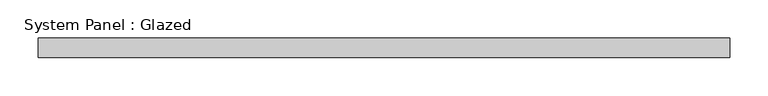
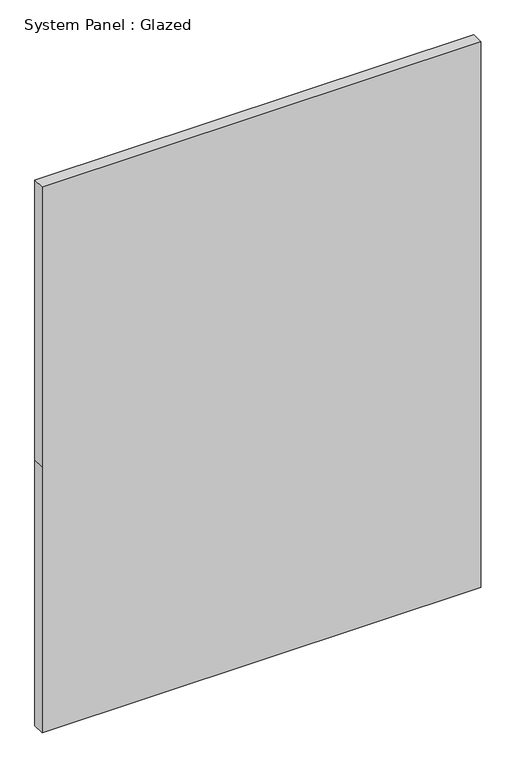
"""IFC4 building model written with IfcOpenShell, lengths in millimetres: plate geometry, System Panel : Glazed."""

import ifcopenshell
import ifcopenshell.guid

model = None  # the IFC model being written
_history = None  # IfcOwnerHistory: only IFC2X3 demands one
_inside = {}  # id of a spatial element -> (the spatial element, [elements in it])
_under = {}  # id of a project, library or spatial element -> (it, [spatial elements below it])
_declared = {}  # id of a project -> (the project, [libraries it declares])
_typed = {}  # id of a type object -> (the type object, [elements of that type])
_made_of = {}  # id of a material, layer set ... -> (it, [elements and type objects made of it])


def new_model(schema):
    """Start an empty IFC model of exactly this schema.

    Asked for "IFC4X3", IfcOpenShell would pick the latest addendum, in which some entities
    have other attributes; the version numbers below select the first issue.
    IFC2X3 requires an IfcOwnerHistory on every rooted entity: one is made here for all.
    """
    global model, _history
    if schema == "IFC4X3":
        model = ifcopenshell.file(schema_version=(4, 3, 0, 0))
    else:
        model = ifcopenshell.file(schema=schema)
    _inside.clear()
    _under.clear()
    _declared.clear()
    _typed.clear()
    _made_of.clear()
    _history = None
    if model.schema == "IFC2X3":
        org = make("IfcOrganization", Name="unknown")
        user = make(
            "IfcPersonAndOrganization",
            ThePerson=make("IfcPerson", FamilyName="unknown"),
            TheOrganization=org,
        )
        app = make(
            "IfcApplication",
            ApplicationDeveloper=org,
            Version="unknown",
            ApplicationFullName="unknown",
            ApplicationIdentifier="unknown",
        )
        _history = make(
            "IfcOwnerHistory",
            OwningUser=user,
            OwningApplication=app,
            ChangeAction="ADDED",
            CreationDate=0,
        )
    return model


def make(cls, **values):
    """One entity of the class cls with the attributes given. An attribute that is None is left unset."""
    return model.create_entity(
        cls, **{name: value for name, value in values.items() if value is not None}
    )


def rooted(cls, **values):
    """An entity with a GlobalId (a new one), such as an element, a storey or a relation."""
    return make(cls, GlobalId=ifcopenshell.guid.new(), OwnerHistory=_history, **values)


def si_unit(unit_type, name, prefix=None):
    """IfcSIUnit, for example si_unit("LENGTHUNIT", "METRE", prefix="MILLI")."""
    return make("IfcSIUnit", UnitType=unit_type, Prefix=prefix, Name=name)


def assignment(units):
    """IfcUnitAssignment: the units of a project."""
    return None if units is None else make("IfcUnitAssignment", Units=units)


def point(xyz):
    """IfcCartesianPoint."""
    return None if xyz is None else make("IfcCartesianPoint", Coordinates=xyz)


def direction(xyz):
    """IfcDirection."""
    return None if xyz is None else make("IfcDirection", DirectionRatios=xyz)


def frame(location, z_axis=None, x_axis=None):
    """IfcAxis2Placement3D, a coordinate frame: its origin and axes. An axis left out is left unset."""
    return make(
        "IfcAxis2Placement3D",
        Location=point(location),
        Axis=direction(z_axis),
        RefDirection=direction(x_axis),
    )


def origin():
    """The frame at (0, 0, 0) with its axes left unset."""
    return frame((0.0, 0.0, 0.0))


def place(relative_to, where):
    """IfcLocalPlacement: puts the frame where relative to a parent placement (None: the world)."""
    return make(
        "IfcLocalPlacement", PlacementRelTo=relative_to, RelativePlacement=where
    )


def context(
    kind, dimensions, precision=None, world=None, true_north=None, identifier=None
):
    """IfcGeometricRepresentationContext, for example the 3D "Model" context."""
    return make(
        "IfcGeometricRepresentationContext",
        ContextIdentifier=identifier,
        ContextType=kind,
        CoordinateSpaceDimension=dimensions,
        Precision=precision,
        WorldCoordinateSystem=world,
        TrueNorth=true_north,
    )


def project(units=None, contexts=None):
    """IfcProject with its units and contexts."""
    return rooted(
        "IfcProject",
        Name="project",
        RepresentationContexts=contexts,
        UnitsInContext=assignment(units),
    )


def spatial(cls, under=None, at=None, **own):
    """A site, building, storey or space (cls), placed at a placement, below another one or the project."""
    s = rooted(cls, ObjectPlacement=at, **own)
    if under is not None:
        _under.setdefault(under.id(), (under, []))[1].append(s)
    return s


def polyline(points):
    """IfcPolyline through the points."""
    return make("IfcPolyline", Points=[point(p) for p in points])


def outline(outer, holes=None, kind="AREA"):
    """IfcArbitraryClosedProfileDef: a profile drawn as a closed curve; with holes, ...WithVoids."""
    if holes is None:
        return make("IfcArbitraryClosedProfileDef", ProfileType=kind, OuterCurve=outer)
    return make(
        "IfcArbitraryProfileDefWithVoids",
        ProfileType=kind,
        OuterCurve=outer,
        InnerCurves=holes,
    )


def extrude(swept, where, along, depth):
    """IfcExtrudedAreaSolid: the profile swept, set in the frame where, extruded along a direction by depth."""
    return make(
        "IfcExtrudedAreaSolid",
        SweptArea=swept,
        Position=where,
        ExtrudedDirection=direction(along),
        Depth=depth,
    )


def shape(context_of_items, identifier, shape_type, items):
    """IfcShapeRepresentation: the items that make up one representation, for example the "Body"."""
    return make(
        "IfcShapeRepresentation",
        ContextOfItems=context_of_items,
        RepresentationIdentifier=identifier,
        RepresentationType=shape_type,
        Items=items,
    )


def source(mapping_origin, context_of_items, identifier, shape_type, items):
    """IfcRepresentationMap: a shape defined once, which mapped items show again and again."""
    return make(
        "IfcRepresentationMap",
        MappingOrigin=mapping_origin,
        MappedRepresentation=shape(context_of_items, identifier, shape_type, items),
    )


def transform(
    local_origin,
    x_axis=None,
    y_axis=None,
    z_axis=None,
    scale=None,
    scale2=None,
    scale3=None,
    uniform=True,
):
    """IfcCartesianTransformationOperator3D, or its non-uniform kind. x_axis, y_axis, z_axis: its Axis1, 2, 3."""
    if uniform:
        return make(
            "IfcCartesianTransformationOperator3D",
            Axis1=direction(x_axis),
            Axis2=direction(y_axis),
            LocalOrigin=point(local_origin),
            Scale=scale,
            Axis3=direction(z_axis),
        )
    return make(
        "IfcCartesianTransformationOperator3DnonUniform",
        Axis1=direction(x_axis),
        Axis2=direction(y_axis),
        LocalOrigin=point(local_origin),
        Scale=scale,
        Axis3=direction(z_axis),
        Scale2=scale2,
        Scale3=scale3,
    )


def mapped(mapping_source, mapping_target):
    """IfcMappedItem: shows the shape of a source again, moved by a transform."""
    return make(
        "IfcMappedItem", MappingSource=mapping_source, MappingTarget=mapping_target
    )


def made_of(thing, what):
    """Note that an element or type object is made of a material, layer set ...; save() writes the relation."""
    if what is not None:
        _made_of.setdefault(what.id(), (what, []))[1].append(thing)
    return thing


def element(
    cls,
    number,
    at=None,
    inside=None,
    cuts=None,
    type_object=None,
    material=None,
    context=None,
    identifier="Body",
    shape_type=None,
    held_by="IfcProductDefinitionShape",
    body=None,
    shapes=None,
    **own,
):
    """One element of the class cls, such as IfcWall. Its Tag is "e" and its number.

    at: its placement. inside: the storey or other place that contains it. cuts: it is an
    opening in that element (IfcRelVoidsElement). A single representation is given by context,
    identifier, shape_type and body (its items); several are given by shapes. held_by: the class
    of the entity that holds the representations. save() writes the other relations.
    """
    e = rooted(cls, Tag="e%d" % number, ObjectPlacement=at, **own)
    if body is not None:
        shapes = [shape(context, identifier, shape_type, body)]
    if shapes is not None:
        e.Representation = make(held_by, Representations=shapes)
    if inside is not None:
        _inside.setdefault(inside.id(), (inside, []))[1].append(e)
    if cuts is not None:
        rooted(
            "IfcRelVoidsElement", RelatingBuildingElement=cuts, RelatedOpeningElement=e
        )
    if type_object is not None:
        _typed.setdefault(type_object.id(), (type_object, []))[1].append(e)
    return made_of(e, material)


def aggregate(whole, parts):
    """IfcRelAggregates: a whole, such as a stair, and the parts it consists of."""
    return rooted("IfcRelAggregates", RelatingObject=whole, RelatedObjects=parts)


def save(model, path):
    """Write the relations noted so far, then the file.

    IfcRelAggregates (storeys below a building ...), IfcRelContainedInSpatialStructure (elements
    in a storey), IfcRelDefinesByType, IfcRelAssociatesMaterial and IfcRelDeclares: one each for
    every whole, place, type object, material and project.
    """
    for whole, parts in _under.values():
        aggregate(whole, parts)
    for where, things in _inside.values():
        rooted(
            "IfcRelContainedInSpatialStructure",
            RelatedElements=things,
            RelatingStructure=where,
        )
    for kind, things in _typed.values():
        rooted("IfcRelDefinesByType", RelatedObjects=things, RelatingType=kind)
    for what, things in _made_of.values():
        rooted("IfcRelAssociatesMaterial", RelatedObjects=things, RelatingMaterial=what)
    for by, libraries in _declared.values():
        rooted("IfcRelDeclares", RelatingContext=by, RelatedDefinitions=libraries)
    model.write(path)


def system_panel_glazed_d47dd273(model_context):
    return source(origin(), model_context, "Body", "SweptSolid", [
        extrude(outline(polyline([(0.0, -451.3791667), (0.0, 451.3791667), (577.85, 451.3791667), (1187.45, 451.3791667), (1187.45, -451.3791667), (577.85, -451.3791667), (0.0, -451.3791667)])), frame((0.0, -44.45, 0.0), z_axis=(0.0, 1.0, 0.0), x_axis=(0.0, 0.0, 1.0)), (0.0, 0.0, 1.0), 25.4),
    ])


if __name__ == "__main__":
    model = new_model("IFC4")
    model_context = context("Model", 3, world=origin())
    ifc_project = project(units=[si_unit("LENGTHUNIT", "METRE", prefix="MILLI")], contexts=[model_context])
    site = spatial("IfcSite", under=ifc_project)
    building = spatial("IfcBuilding", under=site)
    placement = place(None, origin())
    system_panel_glazed_shape = system_panel_glazed_d47dd273(model_context)
    element("IfcPlate", 1, ObjectType="System Panel : Glazed", at=placement, inside=building, context=model_context, shape_type="MappedRepresentation", body=[
        mapped(system_panel_glazed_shape, transform((0.0, 0.0, 0.0), x_axis=(1.0, 0.0, 0.0), y_axis=(0.0, 1.0, 0.0), z_axis=(0.0, 0.0, 1.0))),
    ])
    save(model, "model.ifc")

# Revit data of these elements
# Element 1 (IfcPlate, "System Panel : Glazed")
#   Materials on its faces: "Glass"
# Materials
#   "Glass": class "Unassigned", colour RGB 0 0 255, transparency 0.75
